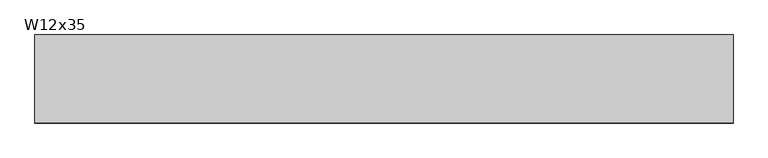
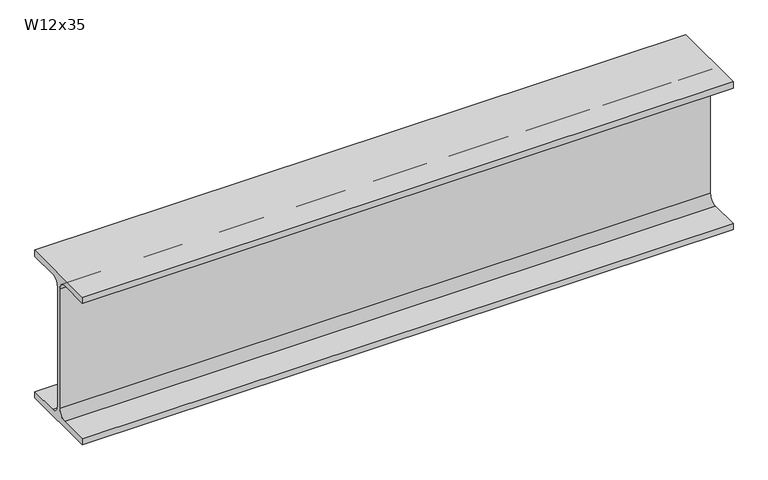
"""IFC4 building model written with IfcOpenShell, lengths in millimetres: beam geometry, RME W-Wide Flange : W12x35."""

from ifc_helpers import new_model, si_unit, point, frame, frame_2d, origin, place, context, project, spatial, polyline, circle_curve, trimmed, segment, composite_curve, outline, extrude, source, transform, mapped, element, save


def w12x35_ceaafe31(model_context):
    return source(origin(), model_context, "Body", "SweptSolid", [
        extrude(outline(composite_curve([segment(polyline([(83.312, -145.542), (83.312, -158.75), (-83.312, -158.75), (-83.312, -145.542), (-20.7645, -145.542)]), True, "CONTINUOUS"), segment(trimmed(circle_curve(frame_2d((-20.7645, -128.5875)), 16.9545), [point((-20.7645, -145.542))], [point((-3.81, -128.5875))], True, "CARTESIAN"), True, "CONTINUOUS"), segment(polyline([(-3.81, -128.5875), (-3.81, 128.5875)]), True, "CONTINUOUS"), segment(trimmed(circle_curve(frame_2d((-20.7645, 128.5875)), 16.9545), [point((-3.81, 128.5875))], [point((-20.7645, 145.542))], True, "CARTESIAN"), True, "CONTINUOUS"), segment(polyline([(-20.7645, 145.542), (-83.312, 145.542), (-83.312, 158.75), (83.312, 158.75), (83.312, 145.542), (20.7645, 145.542)]), True, "CONTINUOUS"), segment(trimmed(circle_curve(frame_2d((20.7645, 128.5875)), 16.9545), [point((20.7645, 145.542))], [point((3.81, 128.5875))], True, "CARTESIAN"), True, "CONTINUOUS"), segment(polyline([(3.81, 128.5875), (3.81, -128.5875)]), True, "CONTINUOUS"), segment(trimmed(circle_curve(frame_2d((20.7645, -128.5875)), 16.9545), [point((3.81, -128.5875))], [point((20.7645, -145.542))], True, "CARTESIAN"), True, "CONTINUOUS"), segment(polyline([(20.7645, -145.542), (83.312, -145.542)]), True, "CONTINUOUS")], self_intersect=False)), frame((-660.4, 0.0, 0.0), z_axis=(1.0, 0.0, 0.0), x_axis=(0.0, 1.0, 0.0)), (0.0, 0.0, 1.0), 1320.8),
    ])


if __name__ == "__main__":
    model = new_model("IFC4")
    model_context = context("Model", 3, world=origin())
    ifc_project = project(units=[si_unit("LENGTHUNIT", "METRE", prefix="MILLI")], contexts=[model_context])
    site = spatial("IfcSite", under=ifc_project)
    building = spatial("IfcBuilding", under=site)
    placement = place(None, origin())
    w12x35_shape = w12x35_ceaafe31(model_context)
    element("IfcBeam", 1, ObjectType="RME W-Wide Flange : W12x35", at=placement, inside=building, context=model_context, shape_type="MappedRepresentation", body=[
        mapped(w12x35_shape, transform((0.0, 0.0, 0.0), x_axis=(1.0, 0.0, 0.0), y_axis=(0.0, 1.0, 0.0), z_axis=(0.0, 0.0, 1.0))),
    ])
    save(model, "model.ifc")

# Revit data of these elements
# Type "RME W-Wide Flange : W12x35"
#   WELD P [instance default] = ""
#   WELD LE [instance default] = ""
#   WELD D [instance default] = ""
#   TOP SECTION SIZE [instance default] = ""
#   TOP SECTION LENGTH [instance default] = ""
#   REMARKS [instance default] = ""
#   REINF TYPE [instance default] = ""
#   Nominal Size = "W24"
#   End Bearing Capacity [instance default] = ""
#   BOT SECTION SIZE [instance default] = ""
#   BOT SECTION LENGTH [instance default] = ""
#   Assembly Code = "B10"
#   W = 35
#   Start Extension Calculation [instance default] = 10' - 0"
#   Start Extension [instance default] = -0' - 0 1/2"
#   End Extension Calculation [instance default] = 10' - 0"
#   End Extension [instance default] = -0' - 0 1/2"
#   Length [instance default] = 5' - 0"
#   bf = 0' - 6.56"
#   d = 1' - 0 1/2"
#   k = 0' - 1 3/16"
#   k2 = 0' - 0.6675"
#   tf = 0' - 0.52"
#   tw = 0' - 0.3"
#   A = 0.0715278 SF
#   Structural Material [instance default] = Metal - Steel - ASTM A992
# Element 1 (IfcBeam, "RME W-Wide Flange : W12x35")
#   Length = 4' - 4"
#   Materials on its faces: "Metal - Steel - ASTM A992"
# Materials
#   "Metal - Steel - ASTM A992": class "Metal", colour RGB 255 128 0, transparency 0
